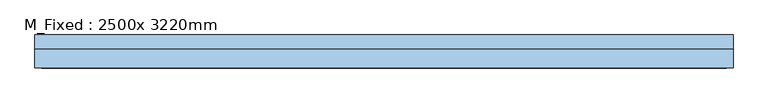
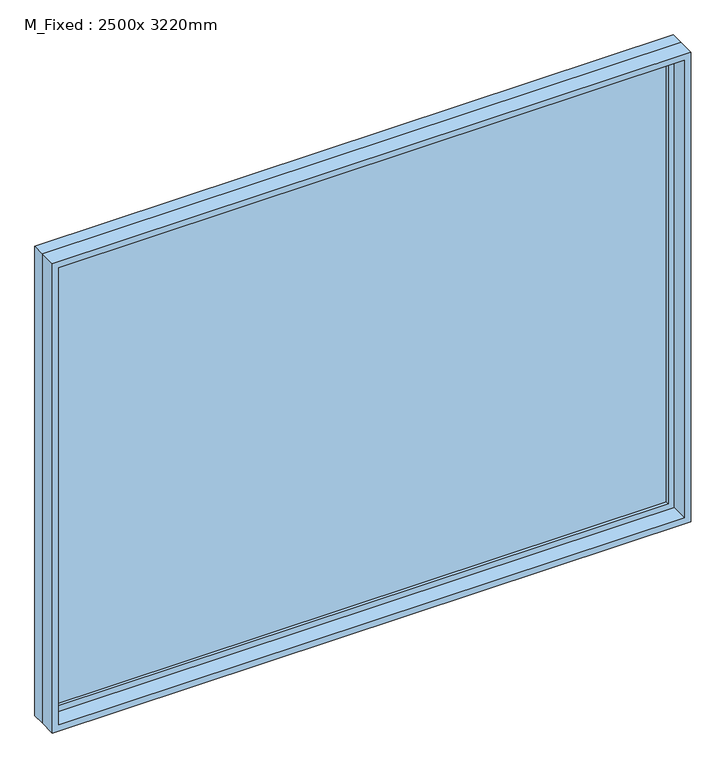
"""IFC4 building model written with IfcOpenShell, lengths in millimetres: window geometry, M_Fixed : 2500x 3220mm."""

import ifcopenshell
import ifcopenshell.guid

model = None  # the IFC model being written
_history = None  # IfcOwnerHistory: only IFC2X3 demands one
_inside = {}  # id of a spatial element -> (the spatial element, [elements in it])
_under = {}  # id of a project, library or spatial element -> (it, [spatial elements below it])
_declared = {}  # id of a project -> (the project, [libraries it declares])
_typed = {}  # id of a type object -> (the type object, [elements of that type])
_made_of = {}  # id of a material, layer set ... -> (it, [elements and type objects made of it])


def new_model(schema):
    """Start an empty IFC model of exactly this schema.

    Asked for "IFC4X3", IfcOpenShell would pick the latest addendum, in which some entities
    have other attributes; the version numbers below select the first issue.
    IFC2X3 requires an IfcOwnerHistory on every rooted entity: one is made here for all.
    """
    global model, _history
    if schema == "IFC4X3":
        model = ifcopenshell.file(schema_version=(4, 3, 0, 0))
    else:
        model = ifcopenshell.file(schema=schema)
    _inside.clear()
    _under.clear()
    _declared.clear()
    _typed.clear()
    _made_of.clear()
    _history = None
    if model.schema == "IFC2X3":
        org = make("IfcOrganization", Name="unknown")
        user = make(
            "IfcPersonAndOrganization",
            ThePerson=make("IfcPerson", FamilyName="unknown"),
            TheOrganization=org,
        )
        app = make(
            "IfcApplication",
            ApplicationDeveloper=org,
            Version="unknown",
            ApplicationFullName="unknown",
            ApplicationIdentifier="unknown",
        )
        _history = make(
            "IfcOwnerHistory",
            OwningUser=user,
            OwningApplication=app,
            ChangeAction="ADDED",
            CreationDate=0,
        )
    return model


def make(cls, **values):
    """One entity of the class cls with the attributes given. An attribute that is None is left unset."""
    return model.create_entity(
        cls, **{name: value for name, value in values.items() if value is not None}
    )


def rooted(cls, **values):
    """An entity with a GlobalId (a new one), such as an element, a storey or a relation."""
    return make(cls, GlobalId=ifcopenshell.guid.new(), OwnerHistory=_history, **values)


def si_unit(unit_type, name, prefix=None):
    """IfcSIUnit, for example si_unit("LENGTHUNIT", "METRE", prefix="MILLI")."""
    return make("IfcSIUnit", UnitType=unit_type, Prefix=prefix, Name=name)


def assignment(units):
    """IfcUnitAssignment: the units of a project."""
    return None if units is None else make("IfcUnitAssignment", Units=units)


def point(xyz):
    """IfcCartesianPoint."""
    return None if xyz is None else make("IfcCartesianPoint", Coordinates=xyz)


def direction(xyz):
    """IfcDirection."""
    return None if xyz is None else make("IfcDirection", DirectionRatios=xyz)


def frame(location, z_axis=None, x_axis=None):
    """IfcAxis2Placement3D, a coordinate frame: its origin and axes. An axis left out is left unset."""
    return make(
        "IfcAxis2Placement3D",
        Location=point(location),
        Axis=direction(z_axis),
        RefDirection=direction(x_axis),
    )


def origin():
    """The frame at (0, 0, 0) with its axes left unset."""
    return frame((0.0, 0.0, 0.0))


def place(relative_to, where):
    """IfcLocalPlacement: puts the frame where relative to a parent placement (None: the world)."""
    return make(
        "IfcLocalPlacement", PlacementRelTo=relative_to, RelativePlacement=where
    )


def context(
    kind, dimensions, precision=None, world=None, true_north=None, identifier=None
):
    """IfcGeometricRepresentationContext, for example the 3D "Model" context."""
    return make(
        "IfcGeometricRepresentationContext",
        ContextIdentifier=identifier,
        ContextType=kind,
        CoordinateSpaceDimension=dimensions,
        Precision=precision,
        WorldCoordinateSystem=world,
        TrueNorth=true_north,
    )


def project(units=None, contexts=None):
    """IfcProject with its units and contexts."""
    return rooted(
        "IfcProject",
        Name="project",
        RepresentationContexts=contexts,
        UnitsInContext=assignment(units),
    )


def spatial(cls, under=None, at=None, **own):
    """A site, building, storey or space (cls), placed at a placement, below another one or the project."""
    s = rooted(cls, ObjectPlacement=at, **own)
    if under is not None:
        _under.setdefault(under.id(), (under, []))[1].append(s)
    return s


def polyline(points):
    """IfcPolyline through the points."""
    return make("IfcPolyline", Points=[point(p) for p in points])


def outline(outer, holes=None, kind="AREA"):
    """IfcArbitraryClosedProfileDef: a profile drawn as a closed curve; with holes, ...WithVoids."""
    if holes is None:
        return make("IfcArbitraryClosedProfileDef", ProfileType=kind, OuterCurve=outer)
    return make(
        "IfcArbitraryProfileDefWithVoids",
        ProfileType=kind,
        OuterCurve=outer,
        InnerCurves=holes,
    )


def extrude(swept, where, along, depth):
    """IfcExtrudedAreaSolid: the profile swept, set in the frame where, extruded along a direction by depth."""
    return make(
        "IfcExtrudedAreaSolid",
        SweptArea=swept,
        Position=where,
        ExtrudedDirection=direction(along),
        Depth=depth,
    )


def shape(context_of_items, identifier, shape_type, items):
    """IfcShapeRepresentation: the items that make up one representation, for example the "Body"."""
    return make(
        "IfcShapeRepresentation",
        ContextOfItems=context_of_items,
        RepresentationIdentifier=identifier,
        RepresentationType=shape_type,
        Items=items,
    )


def source(mapping_origin, context_of_items, identifier, shape_type, items):
    """IfcRepresentationMap: a shape defined once, which mapped items show again and again."""
    return make(
        "IfcRepresentationMap",
        MappingOrigin=mapping_origin,
        MappedRepresentation=shape(context_of_items, identifier, shape_type, items),
    )


def transform(
    local_origin,
    x_axis=None,
    y_axis=None,
    z_axis=None,
    scale=None,
    scale2=None,
    scale3=None,
    uniform=True,
):
    """IfcCartesianTransformationOperator3D, or its non-uniform kind. x_axis, y_axis, z_axis: its Axis1, 2, 3."""
    if uniform:
        return make(
            "IfcCartesianTransformationOperator3D",
            Axis1=direction(x_axis),
            Axis2=direction(y_axis),
            LocalOrigin=point(local_origin),
            Scale=scale,
            Axis3=direction(z_axis),
        )
    return make(
        "IfcCartesianTransformationOperator3DnonUniform",
        Axis1=direction(x_axis),
        Axis2=direction(y_axis),
        LocalOrigin=point(local_origin),
        Scale=scale,
        Axis3=direction(z_axis),
        Scale2=scale2,
        Scale3=scale3,
    )


def mapped(mapping_source, mapping_target):
    """IfcMappedItem: shows the shape of a source again, moved by a transform."""
    return make(
        "IfcMappedItem", MappingSource=mapping_source, MappingTarget=mapping_target
    )


def made_of(thing, what):
    """Note that an element or type object is made of a material, layer set ...; save() writes the relation."""
    if what is not None:
        _made_of.setdefault(what.id(), (what, []))[1].append(thing)
    return thing


def element(
    cls,
    number,
    at=None,
    inside=None,
    cuts=None,
    type_object=None,
    material=None,
    context=None,
    identifier="Body",
    shape_type=None,
    held_by="IfcProductDefinitionShape",
    body=None,
    shapes=None,
    **own,
):
    """One element of the class cls, such as IfcWall. Its Tag is "e" and its number.

    at: its placement. inside: the storey or other place that contains it. cuts: it is an
    opening in that element (IfcRelVoidsElement). A single representation is given by context,
    identifier, shape_type and body (its items); several are given by shapes. held_by: the class
    of the entity that holds the representations. save() writes the other relations.
    """
    e = rooted(cls, Tag="e%d" % number, ObjectPlacement=at, **own)
    if body is not None:
        shapes = [shape(context, identifier, shape_type, body)]
    if shapes is not None:
        e.Representation = make(held_by, Representations=shapes)
    if inside is not None:
        _inside.setdefault(inside.id(), (inside, []))[1].append(e)
    if cuts is not None:
        rooted(
            "IfcRelVoidsElement", RelatingBuildingElement=cuts, RelatedOpeningElement=e
        )
    if type_object is not None:
        _typed.setdefault(type_object.id(), (type_object, []))[1].append(e)
    return made_of(e, material)


def aggregate(whole, parts):
    """IfcRelAggregates: a whole, such as a stair, and the parts it consists of."""
    return rooted("IfcRelAggregates", RelatingObject=whole, RelatedObjects=parts)


def save(model, path):
    """Write the relations noted so far, then the file.

    IfcRelAggregates (storeys below a building ...), IfcRelContainedInSpatialStructure (elements
    in a storey), IfcRelDefinesByType, IfcRelAssociatesMaterial and IfcRelDeclares: one each for
    every whole, place, type object, material and project.
    """
    for whole, parts in _under.values():
        aggregate(whole, parts)
    for where, things in _inside.values():
        rooted(
            "IfcRelContainedInSpatialStructure",
            RelatedElements=things,
            RelatingStructure=where,
        )
    for kind, things in _typed.values():
        rooted("IfcRelDefinesByType", RelatedObjects=things, RelatingType=kind)
    for what, things in _made_of.values():
        rooted("IfcRelAssociatesMaterial", RelatedObjects=things, RelatingMaterial=what)
    for by, libraries in _declared.values():
        rooted("IfcRelDeclares", RelatingContext=by, RelatedDefinitions=libraries)
    model.write(path)


def m_fixed_2500x_3220mm_df94f4d0(model_context):
    return source(origin(), model_context, "Body", "SweptSolid", [
        extrude(outline(polyline([(-1546.8, 54.2), (1546.8, 54.2), (1546.8, 42.2), (-1546.8, 42.2), (-1546.8, 54.2)])), frame((0.0, 0.0, 368.0), z_axis=(0.0, 0.0, 1.0), x_axis=(1.0, 0.0, 0.0)), (0.0, 0.0, 1.0), 2374.0),
        extrude(outline(polyline([(2786.0, -1590.8), (324.0, -1590.8), (324.0, 1590.8), (2786.0, 1590.8), (2786.0, -1590.8)]), holes=[polyline([(2742.0, -1546.8), (2742.0, 1546.8), (368.0, 1546.8), (368.0, -1546.8), (2742.0, -1546.8)])]), frame((0.0, 26.2, 0.0), z_axis=(0.0, 1.0, 0.0), x_axis=(0.0, 0.0, 1.0)), (0.0, 0.0, 1.0), 44.0),
        extrude(outline(polyline([(2805.0, -1609.8), (305.0, -1609.8), (305.0, 1609.8), (2805.0, 1609.8), (2805.0, -1609.8)]), holes=[polyline([(2786.0, -1590.8), (2786.0, 1590.8), (324.0, 1590.8), (324.0, -1590.8), (2786.0, -1590.8)])]), frame((0.0, 26.2, 0.0), z_axis=(0.0, 1.0, 0.0), x_axis=(0.0, 0.0, 1.0)), (0.0, 0.0, 1.0), 63.0),
        extrude(outline(polyline([(2805.0, -1609.8), (305.0, -1609.8), (305.0, 1609.8), (2805.0, 1609.8), (2805.0, -1609.8)]), holes=[polyline([(2773.0, -1577.8), (2773.0, 1577.8), (337.0, 1577.8), (337.0, -1577.8), (2773.0, -1577.8)])]), frame((0.0, -63.2, 0.0), z_axis=(0.0, 1.0, 0.0), x_axis=(0.0, 0.0, 1.0)), (0.0, 0.0, 1.0), 89.4),
    ])


if __name__ == "__main__":
    model = new_model("IFC4")
    model_context = context("Model", 3, world=origin())
    ifc_project = project(units=[si_unit("LENGTHUNIT", "METRE", prefix="MILLI")], contexts=[model_context])
    site = spatial("IfcSite", under=ifc_project)
    building = spatial("IfcBuilding", under=site)
    placement = place(None, origin())
    m_fixed_2500x_3220mm_shape = m_fixed_2500x_3220mm_df94f4d0(model_context)
    element("IfcWindow", 1, ObjectType="M_Fixed : 2500x 3220mm", at=placement, inside=building, context=model_context, shape_type="MappedRepresentation", body=[
        mapped(m_fixed_2500x_3220mm_shape, transform((0.0, 0.0, 0.0), x_axis=(1.0, 0.0, 0.0), y_axis=(0.0, 1.0, 0.0), z_axis=(0.0, 0.0, 1.0))),
    ])
    save(model, "model.ifc")

# Revit data of these elements
# Type "M_Fixed : 2500x 3220mm"
#   Type Mark = "26"
#   Height = 2500 mm
#   Default Sill Height = 305 mm
#   Width = 3219.6 mm
#   Window Inset = 19 mm
#   Frame Exterior Material = Sash
#   Frame Interior Material = Sash
#   Glass Pane Material = Glass
#   Sash = Sash
#   Wall Closure = (empty or 0)
# Element 1 (IfcWindow, "M_Fixed : 2500x 3220mm")
#   Materials on its faces: "Sash", "Glass"
# Materials
#   "Sash": class "Wood", colour RGB 136 99 55, transparency 0
#   "Glass": class "Glass", colour RGB 0 128 192, transparency 0.9, Description = "Soda Lime Glass", Cost = 0
